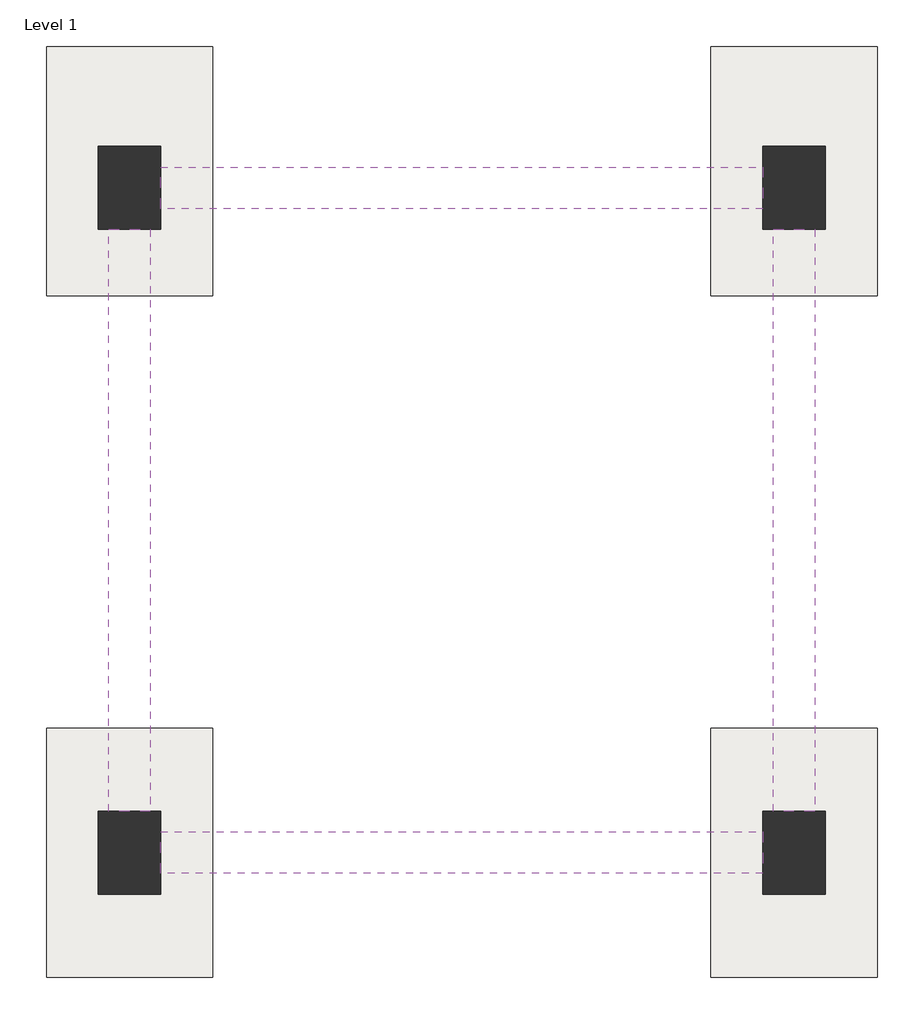
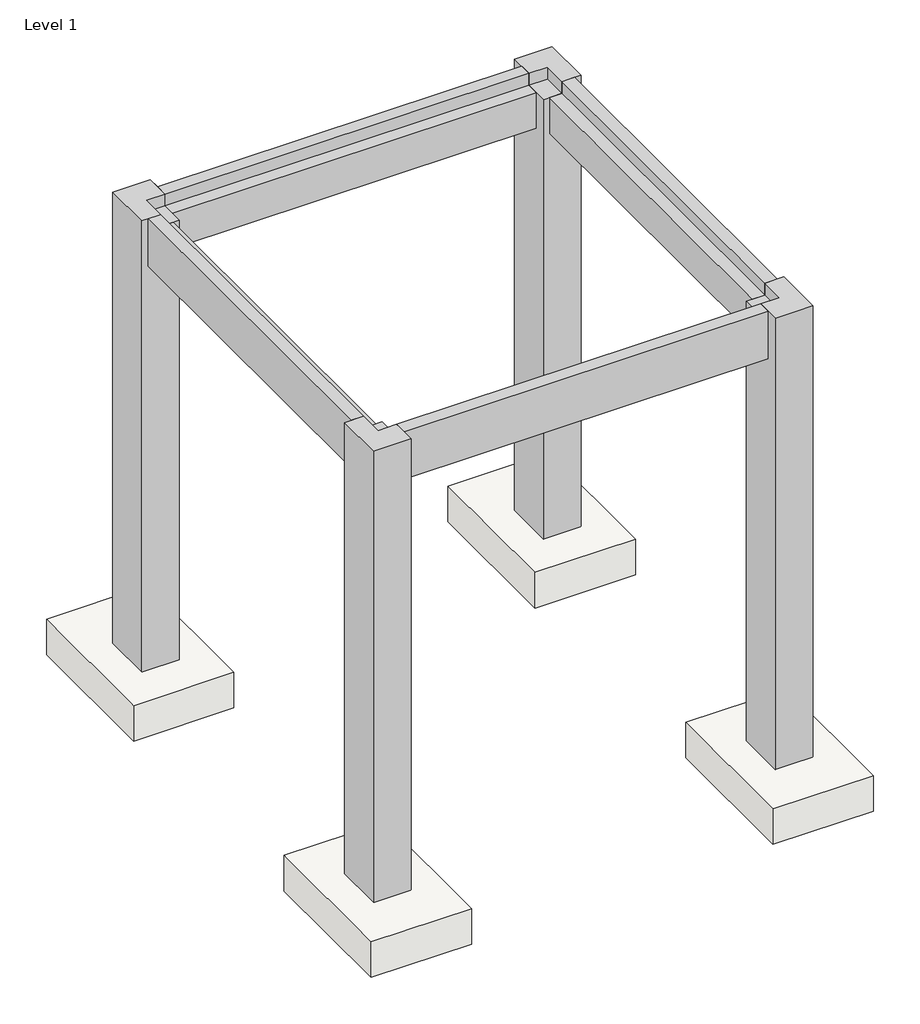
# One storey: 7 columns, 4 beams, 4 slabs.
"""IFC4 building model written with IfcOpenShell, lengths in millimetres."""

import ifcopenshell
import ifcopenshell.guid

model = None  # the IFC model being written
_history = None  # IfcOwnerHistory: only IFC2X3 demands one
_inside = {}  # id of a spatial element -> (the spatial element, [elements in it])
_under = {}  # id of a project, library or spatial element -> (it, [spatial elements below it])
_declared = {}  # id of a project -> (the project, [libraries it declares])
_typed = {}  # id of a type object -> (the type object, [elements of that type])
_made_of = {}  # id of a material, layer set ... -> (it, [elements and type objects made of it])


def new_model(schema):
    """Start an empty IFC model of exactly this schema.

    Asked for "IFC4X3", IfcOpenShell would pick the latest addendum, in which some entities
    have other attributes; the version numbers below select the first issue.
    IFC2X3 requires an IfcOwnerHistory on every rooted entity: one is made here for all.
    """
    global model, _history
    if schema == "IFC4X3":
        model = ifcopenshell.file(schema_version=(4, 3, 0, 0))
    else:
        model = ifcopenshell.file(schema=schema)
    _inside.clear()
    _under.clear()
    _declared.clear()
    _typed.clear()
    _made_of.clear()
    _history = None
    if model.schema == "IFC2X3":
        org = make("IfcOrganization", Name="unknown")
        user = make(
            "IfcPersonAndOrganization",
            ThePerson=make("IfcPerson", FamilyName="unknown"),
            TheOrganization=org,
        )
        app = make(
            "IfcApplication",
            ApplicationDeveloper=org,
            Version="unknown",
            ApplicationFullName="unknown",
            ApplicationIdentifier="unknown",
        )
        _history = make(
            "IfcOwnerHistory",
            OwningUser=user,
            OwningApplication=app,
            ChangeAction="ADDED",
            CreationDate=0,
        )
    return model


def make(cls, **values):
    """One entity of the class cls with the attributes given. An attribute that is None is left unset."""
    return model.create_entity(
        cls, **{name: value for name, value in values.items() if value is not None}
    )


def rooted(cls, **values):
    """An entity with a GlobalId (a new one), such as an element, a storey or a relation."""
    return make(cls, GlobalId=ifcopenshell.guid.new(), OwnerHistory=_history, **values)


def si_unit(unit_type, name, prefix=None):
    """IfcSIUnit, for example si_unit("LENGTHUNIT", "METRE", prefix="MILLI")."""
    return make("IfcSIUnit", UnitType=unit_type, Prefix=prefix, Name=name)


def assignment(units):
    """IfcUnitAssignment: the units of a project."""
    return None if units is None else make("IfcUnitAssignment", Units=units)


def point(xyz):
    """IfcCartesianPoint."""
    return None if xyz is None else make("IfcCartesianPoint", Coordinates=xyz)


def direction(xyz):
    """IfcDirection."""
    return None if xyz is None else make("IfcDirection", DirectionRatios=xyz)


def frame(location, z_axis=None, x_axis=None):
    """IfcAxis2Placement3D, a coordinate frame: its origin and axes. An axis left out is left unset."""
    return make(
        "IfcAxis2Placement3D",
        Location=point(location),
        Axis=direction(z_axis),
        RefDirection=direction(x_axis),
    )


def origin():
    """The frame at (0, 0, 0) with its axes left unset."""
    return frame((0.0, 0.0, 0.0))


def place(relative_to, where):
    """IfcLocalPlacement: puts the frame where relative to a parent placement (None: the world)."""
    return make(
        "IfcLocalPlacement", PlacementRelTo=relative_to, RelativePlacement=where
    )


def context(
    kind, dimensions, precision=None, world=None, true_north=None, identifier=None
):
    """IfcGeometricRepresentationContext, for example the 3D "Model" context."""
    return make(
        "IfcGeometricRepresentationContext",
        ContextIdentifier=identifier,
        ContextType=kind,
        CoordinateSpaceDimension=dimensions,
        Precision=precision,
        WorldCoordinateSystem=world,
        TrueNorth=true_north,
    )


def project(units=None, contexts=None):
    """IfcProject with its units and contexts."""
    return rooted(
        "IfcProject",
        Name="project",
        RepresentationContexts=contexts,
        UnitsInContext=assignment(units),
    )


def spatial(cls, under=None, at=None, **own):
    """A site, building, storey or space (cls), placed at a placement, below another one or the project."""
    s = rooted(cls, ObjectPlacement=at, **own)
    if under is not None:
        _under.setdefault(under.id(), (under, []))[1].append(s)
    return s


def polyline(points):
    """IfcPolyline through the points."""
    return make("IfcPolyline", Points=[point(p) for p in points])


def outline(outer, holes=None, kind="AREA"):
    """IfcArbitraryClosedProfileDef: a profile drawn as a closed curve; with holes, ...WithVoids."""
    if holes is None:
        return make("IfcArbitraryClosedProfileDef", ProfileType=kind, OuterCurve=outer)
    return make(
        "IfcArbitraryProfileDefWithVoids",
        ProfileType=kind,
        OuterCurve=outer,
        InnerCurves=holes,
    )


def extrude(swept, where, along, depth):
    """IfcExtrudedAreaSolid: the profile swept, set in the frame where, extruded along a direction by depth."""
    return make(
        "IfcExtrudedAreaSolid",
        SweptArea=swept,
        Position=where,
        ExtrudedDirection=direction(along),
        Depth=depth,
    )


def faces_of(points, faces, orient=None, outer=None):
    """IfcFace entities. A face is a list of loops; a loop is a list of indices into points, from 0.

    orient and outer hold one flag for each loop. By default every Orientation is true, the
    first loop of a face is its IfcFaceOuterBound and the others are IfcFaceBound.
    """
    made = []
    for i, loops in enumerate(faces):
        bounds = []
        for j, loop in enumerate(loops):
            is_outer = j == 0 if outer is None else outer[i][j]
            bounds.append(
                make(
                    "IfcFaceOuterBound" if is_outer else "IfcFaceBound",
                    Bound=make("IfcPolyLoop", Polygon=[points[k] for k in loop]),
                    Orientation=True if orient is None else orient[i][j],
                )
            )
        made.append(make("IfcFace", Bounds=bounds))
    return made


def faceted_brep(points, faces, orient=None, outer=None, voids=None):
    """IfcFacetedBrep: a solid bounded by flat faces; with voids (closed shells), ...WithVoids."""
    shared = [point(p) for p in points]
    hull = make("IfcClosedShell", CfsFaces=faces_of(shared, faces, orient, outer))
    if voids is None:
        return make("IfcFacetedBrep", Outer=hull)
    return make(
        "IfcFacetedBrepWithVoids",
        Outer=hull,
        Voids=[
            make(cls, CfsFaces=faces_of(shared, fs, o, b)) for cls, fs, o, b in voids
        ],
    )


def shape(context_of_items, identifier, shape_type, items):
    """IfcShapeRepresentation: the items that make up one representation, for example the "Body"."""
    return make(
        "IfcShapeRepresentation",
        ContextOfItems=context_of_items,
        RepresentationIdentifier=identifier,
        RepresentationType=shape_type,
        Items=items,
    )


def source(mapping_origin, context_of_items, identifier, shape_type, items):
    """IfcRepresentationMap: a shape defined once, which mapped items show again and again."""
    return make(
        "IfcRepresentationMap",
        MappingOrigin=mapping_origin,
        MappedRepresentation=shape(context_of_items, identifier, shape_type, items),
    )


def transform(
    local_origin,
    x_axis=None,
    y_axis=None,
    z_axis=None,
    scale=None,
    scale2=None,
    scale3=None,
    uniform=True,
):
    """IfcCartesianTransformationOperator3D, or its non-uniform kind. x_axis, y_axis, z_axis: its Axis1, 2, 3."""
    if uniform:
        return make(
            "IfcCartesianTransformationOperator3D",
            Axis1=direction(x_axis),
            Axis2=direction(y_axis),
            LocalOrigin=point(local_origin),
            Scale=scale,
            Axis3=direction(z_axis),
        )
    return make(
        "IfcCartesianTransformationOperator3DnonUniform",
        Axis1=direction(x_axis),
        Axis2=direction(y_axis),
        LocalOrigin=point(local_origin),
        Scale=scale,
        Axis3=direction(z_axis),
        Scale2=scale2,
        Scale3=scale3,
    )


def mapped(mapping_source, mapping_target):
    """IfcMappedItem: shows the shape of a source again, moved by a transform."""
    return make(
        "IfcMappedItem", MappingSource=mapping_source, MappingTarget=mapping_target
    )


def made_of(thing, what):
    """Note that an element or type object is made of a material, layer set ...; save() writes the relation."""
    if what is not None:
        _made_of.setdefault(what.id(), (what, []))[1].append(thing)
    return thing


def element(
    cls,
    number,
    at=None,
    inside=None,
    cuts=None,
    type_object=None,
    material=None,
    context=None,
    identifier="Body",
    shape_type=None,
    held_by="IfcProductDefinitionShape",
    body=None,
    shapes=None,
    **own,
):
    """One element of the class cls, such as IfcWall. Its Tag is "e" and its number.

    at: its placement. inside: the storey or other place that contains it. cuts: it is an
    opening in that element (IfcRelVoidsElement). A single representation is given by context,
    identifier, shape_type and body (its items); several are given by shapes. held_by: the class
    of the entity that holds the representations. save() writes the other relations.
    """
    e = rooted(cls, Tag="e%d" % number, ObjectPlacement=at, **own)
    if body is not None:
        shapes = [shape(context, identifier, shape_type, body)]
    if shapes is not None:
        e.Representation = make(held_by, Representations=shapes)
    if inside is not None:
        _inside.setdefault(inside.id(), (inside, []))[1].append(e)
    if cuts is not None:
        rooted(
            "IfcRelVoidsElement", RelatingBuildingElement=cuts, RelatedOpeningElement=e
        )
    if type_object is not None:
        _typed.setdefault(type_object.id(), (type_object, []))[1].append(e)
    return made_of(e, material)


def aggregate(whole, parts):
    """IfcRelAggregates: a whole, such as a stair, and the parts it consists of."""
    return rooted("IfcRelAggregates", RelatingObject=whole, RelatedObjects=parts)


def save(model, path):
    """Write the relations noted so far, then the file.

    IfcRelAggregates (storeys below a building ...), IfcRelContainedInSpatialStructure (elements
    in a storey), IfcRelDefinesByType, IfcRelAssociatesMaterial and IfcRelDeclares: one each for
    every whole, place, type object, material and project.
    """
    for whole, parts in _under.values():
        aggregate(whole, parts)
    for where, things in _inside.values():
        rooted(
            "IfcRelContainedInSpatialStructure",
            RelatedElements=things,
            RelatingStructure=where,
        )
    for kind, things in _typed.values():
        rooted("IfcRelDefinesByType", RelatedObjects=things, RelatingType=kind)
    for what, things in _made_of.values():
        rooted("IfcRelAssociatesMaterial", RelatedObjects=things, RelatingMaterial=what)
    for by, libraries in _declared.values():
        rooted("IfcRelDeclares", RelatingContext=by, RelatedDefinitions=libraries)
    model.write(path)


def slab_5ba74754(model_context):
    return source(origin(), model_context, "Body", "SweptSolid", [
        extrude(outline(polyline([(609.6, 914.4), (609.6, -914.4), (-609.6, -914.4), (-609.6, 914.4), (609.6, 914.4)])), frame((0.0, 0.0, -457.2), z_axis=(0.0, 0.0, 1.0), x_axis=(1.0, 0.0, 0.0)), (0.0, 0.0, 1.0), 457.2),
    ])


model = new_model("IFC4")

# Units and contexts
model_context = context("Model", 3, world=origin())
ifc_project = project(units=[si_unit("LENGTHUNIT", "METRE", prefix="MILLI")], contexts=[model_context])

# Site, building, storey
site = spatial("IfcSite", under=ifc_project)
building = spatial("IfcBuilding", under=site)
storey = spatial("IfcBuildingStorey", under=building, Name="Level 1", Elevation=0.0)

# Beams
placement = place(None, origin())
element("IfcBeam", 1, ObjectType="Concrete-Rectangular Beam : 12 x 24", at=placement, inside=storey, context=model_context, shape_type="SweptSolid", body=[
    extrude(outline(polyline([(786.0323826, 2438.4), (786.0323826, 3048.0), (938.4323826, 3048.0), (938.4323826, 2895.6), (1090.8323826, 2895.6), (1090.8323826, 2438.4), (786.0323826, 2438.4)])), frame((-11045.0800525, 0.0, 0.0), z_axis=(1.0, 0.0, 0.0), x_axis=(0.0, 1.0, 0.0)), (0.0, 0.0, 1.0), 4419.6),
])
element("IfcBeam", 2, ObjectType="Concrete-Rectangular Beam : 12 x 24", at=placement, inside=storey, context=model_context, shape_type="SweptSolid", body=[
    extrude(outline(polyline([(5967.6323826, 3048.0), (5967.6323826, 2438.4), (5662.8323826, 2438.4), (5662.8323826, 2895.6), (5815.2323826, 2895.6), (5815.2323826, 3048.0), (5967.6323826, 3048.0)])), frame((-11045.0800525, 0.0, 0.0), z_axis=(1.0, 0.0, 0.0), x_axis=(0.0, 1.0, 0.0)), (0.0, 0.0, 1.0), 4419.6),
])
element("IfcBeam", 3, ObjectType="Concrete-Rectangular Beam : 12 x 24", at=placement, inside=storey, context=model_context, shape_type="SweptSolid", body=[
    extrude(outline(polyline([(2438.4, -11426.0800525), (2438.4, -11121.2800525), (2895.6, -11121.2800525), (2895.6, -11273.6800525), (3048.0, -11273.6800525), (3048.0, -11426.0800525), (2438.4, -11426.0800525)])), frame((0.0, 1243.2323826, 0.0), z_axis=(0.0, 1.0, 0.0), x_axis=(0.0, 0.0, 1.0)), (0.0, 0.0, 1.0), 4267.2),
])
element("IfcBeam", 4, ObjectType="Concrete-Rectangular Beam : 12 x 24", at=placement, inside=storey, context=model_context, shape_type="SweptSolid", body=[
    extrude(outline(polyline([(2438.4, -6244.4800525), (3048.0, -6244.4800525), (3048.0, -6396.8800525), (2895.6, -6396.8800525), (2895.6, -6549.2800525), (2438.4, -6549.2800525), (2438.4, -6244.4800525)])), frame((0.0, 1243.2323826, 0.0), z_axis=(0.0, 1.0, 0.0), x_axis=(0.0, 0.0, 1.0)), (0.0, 0.0, 1.0), 4267.2),
])

# Columns
element("IfcColumn", 5, ObjectType="Concrete-Rectangular-Column : 18 x 24", at=placement, inside=storey, context=model_context, shape_type="Brep", body=[
    faceted_brep([(-11045.0800525, 6120.0323826, 3048.0), (-11502.2800525, 6120.0323826, 3048.0), (-11502.2800525, 5510.4323826, 3048.0), (-11273.6800525, 5510.4323826, 3048.0), (-11273.6800525, 5815.2323826, 3048.0), (-11045.0800525, 5815.2323826, 3048.0), (-11045.0800525, 6120.0323826, -2743.2), (-11045.0800525, 5510.4323826, -2743.2), (-11502.2800525, 5510.4323826, -2743.2), (-11502.2800525, 6120.0323826, -2743.2), (-11045.0800525, 5510.4323826, 2895.6), (-11273.6800525, 5510.4323826, 2895.6), (-11045.0800525, 5815.2323826, 2895.6), (-11273.6800525, 5815.2323826, 2895.6)], [[[0, 1, 2, 3, 4, 5]], [[6, 7, 8, 9]], [[1, 0, 6, 9]], [[2, 1, 9, 8]], [[8, 7, 10, 11, 3, 2]], [[7, 6, 0, 5, 12, 10]], [[13, 11, 10, 12]], [[4, 13, 12, 5]], [[13, 4, 3, 11]]]),
])
element("IfcColumn", 6, ObjectType="Concrete-Rectangular-Column : 18 x 24", at=placement, inside=storey, context=model_context, shape_type="Brep", body=[
    faceted_brep([(-6168.2800525, 6120.0323826, 3048.0), (-6625.4800525, 6120.0323826, 3048.0), (-6625.4800525, 5815.2323826, 3048.0), (-6396.8800525, 5815.2323826, 3048.0), (-6396.8800525, 5510.4323826, 3048.0), (-6168.2800525, 5510.4323826, 3048.0), (-6168.2800525, 6120.0323826, -2743.2), (-6168.2800525, 5510.4323826, -2743.2), (-6625.4800525, 5510.4323826, -2743.2), (-6625.4800525, 6120.0323826, -2743.2), (-6625.4800525, 5510.4323826, 2895.6), (-6625.4800525, 5815.2323826, 2895.6), (-6396.8800525, 5510.4323826, 2895.6), (-6396.8800525, 5815.2323826, 2895.6)], [[[0, 1, 2, 3, 4, 5]], [[6, 7, 8, 9]], [[1, 0, 6, 9]], [[9, 8, 10, 11, 2, 1]], [[8, 7, 5, 4, 12, 10]], [[0, 5, 7, 6]], [[12, 13, 11, 10]], [[13, 3, 2, 11]], [[3, 13, 12, 4]]]),
])
element("IfcColumn", 7, ObjectType="Concrete-Rectangular-Column : 18 x 24", at=placement, inside=storey, context=model_context, shape_type="Brep", body=[
    faceted_brep([(-11045.0800525, 6120.0323826, 3048.0), (-11502.2800525, 6120.0323826, 3048.0), (-11502.2800525, 5510.4323826, 3048.0), (-11426.0800525, 5510.4323826, 3048.0), (-11273.6800525, 5510.4323826, 3048.0), (-11273.6800525, 5815.2323826, 3048.0), (-11045.0800525, 5815.2323826, 3048.0), (-11045.0800525, 5967.6323826, 3048.0), (-11045.0800525, 6120.0323826, -2743.2), (-11045.0800525, 5510.4323826, -2743.2), (-11502.2800525, 5510.4323826, -2743.2), (-11502.2800525, 6120.0323826, -2743.2), (-11045.0800525, 5510.4323826, 2895.6), (-11121.2800525, 5510.4323826, 2895.6), (-11273.6800525, 5510.4323826, 2895.6), (-11045.0800525, 5815.2323826, 2895.6), (-11045.0800525, 5662.8323826, 2895.6), (-11273.6800525, 5815.2323826, 2895.6)], [[[0, 1, 2, 3, 4, 5, 6, 7]], [[8, 9, 10, 11]], [[1, 0, 8, 11]], [[2, 1, 11, 10]], [[10, 9, 12, 13, 14, 4, 3, 2]], [[9, 8, 0, 7, 6, 15, 16, 12]], [[17, 14, 13, 12, 16, 15]], [[5, 17, 15, 6]], [[17, 5, 4, 14]]]),
])
element("IfcColumn", 8, ObjectType="Concrete-Rectangular-Column : 18 x 24", at=placement, inside=storey, context=model_context, shape_type="Brep", body=[
    faceted_brep([(-11045.0800525, 6120.0323826, 3048.0), (-11502.2800525, 6120.0323826, 3048.0), (-11502.2800525, 5510.4323826, 3048.0), (-11426.0800525, 5510.4323826, 3048.0), (-11273.6800525, 5510.4323826, 3048.0), (-11273.6800525, 5815.2323826, 3048.0), (-11045.0800525, 5815.2323826, 3048.0), (-11045.0800525, 5967.6323826, 3048.0), (-11045.0800525, 6120.0323826, -2743.2), (-11045.0800525, 5510.4323826, -2743.2), (-11502.2800525, 5510.4323826, -2743.2), (-11502.2800525, 6120.0323826, -2743.2), (-11045.0800525, 5510.4323826, 2895.6), (-11121.2800525, 5510.4323826, 2895.6), (-11273.6800525, 5510.4323826, 2895.6), (-11045.0800525, 5815.2323826, 2895.6), (-11045.0800525, 5662.8323826, 2895.6), (-11273.6800525, 5815.2323826, 2895.6)], [[[0, 1, 2, 3, 4, 5, 6, 7]], [[8, 9, 10, 11]], [[1, 0, 8, 11]], [[2, 1, 11, 10]], [[10, 9, 12, 13, 14, 4, 3, 2]], [[9, 8, 0, 7, 6, 15, 16, 12]], [[17, 14, 13, 12, 16, 15]], [[5, 17, 15, 6]], [[17, 5, 4, 14]]]),
])
element("IfcColumn", 9, ObjectType="Concrete-Rectangular-Column : 18 x 24", at=placement, inside=storey, context=model_context, shape_type="Brep", body=[
    faceted_brep([(-11045.0800525, 6120.0323826, 3048.0), (-11502.2800525, 6120.0323826, 3048.0), (-11502.2800525, 5510.4323826, 3048.0), (-11426.0800525, 5510.4323826, 3048.0), (-11273.6800525, 5510.4323826, 3048.0), (-11273.6800525, 5815.2323826, 3048.0), (-11045.0800525, 5815.2323826, 3048.0), (-11045.0800525, 5967.6323826, 3048.0), (-11045.0800525, 6120.0323826, -2743.2), (-11045.0800525, 5510.4323826, -2743.2), (-11502.2800525, 5510.4323826, -2743.2), (-11502.2800525, 6120.0323826, -2743.2), (-11045.0800525, 5510.4323826, 2895.6), (-11121.2800525, 5510.4323826, 2895.6), (-11273.6800525, 5510.4323826, 2895.6), (-11045.0800525, 5815.2323826, 2895.6), (-11045.0800525, 5662.8323826, 2895.6), (-11273.6800525, 5815.2323826, 2895.6)], [[[0, 1, 2, 3, 4, 5, 6, 7]], [[8, 9, 10, 11]], [[1, 0, 8, 11]], [[2, 1, 11, 10]], [[10, 9, 12, 13, 14, 4, 3, 2]], [[9, 8, 0, 7, 6, 15, 16, 12]], [[17, 14, 13, 12, 16, 15]], [[5, 17, 15, 6]], [[17, 5, 4, 14]]]),
])
element("IfcColumn", 10, ObjectType="Concrete-Rectangular-Column : 18 x 24", at=placement, inside=storey, context=model_context, shape_type="Brep", body=[
    faceted_brep([(-11502.2800525, 1243.2323826, 3048.0), (-11502.2800525, 633.6323826, 3048.0), (-11045.0800525, 633.6323826, 3048.0), (-11045.0800525, 938.4323826, 3048.0), (-11273.6800525, 938.4323826, 3048.0), (-11273.6800525, 1243.2323826, 3048.0), (-11045.0800525, 1243.2323826, -2743.2), (-11045.0800525, 633.6323826, -2743.2), (-11502.2800525, 633.6323826, -2743.2), (-11502.2800525, 1243.2323826, -2743.2), (-11273.6800525, 1243.2323826, 2895.6), (-11045.0800525, 1243.2323826, 2895.6), (-11045.0800525, 938.4323826, 2895.6), (-11273.6800525, 938.4323826, 2895.6)], [[[0, 1, 2, 3, 4, 5]], [[6, 7, 8, 9]], [[6, 9, 0, 5, 10, 11]], [[1, 0, 9, 8]], [[2, 1, 8, 7]], [[7, 6, 11, 12, 3, 2]], [[10, 13, 12, 11]], [[13, 4, 3, 12]], [[4, 13, 10, 5]]]),
])
element("IfcColumn", 11, ObjectType="Concrete-Rectangular-Column : 18 x 24", at=placement, inside=storey, context=model_context, shape_type="Brep", body=[
    faceted_brep([(-6625.4800525, 633.6323826, 3048.0), (-6168.2800525, 633.6323826, 3048.0), (-6168.2800525, 1243.2323826, 3048.0), (-6396.8800525, 1243.2323826, 3048.0), (-6396.8800525, 938.4323826, 3048.0), (-6625.4800525, 938.4323826, 3048.0), (-6168.2800525, 1243.2323826, -2743.2), (-6168.2800525, 633.6323826, -2743.2), (-6625.4800525, 633.6323826, -2743.2), (-6625.4800525, 1243.2323826, -2743.2), (-6625.4800525, 1243.2323826, 2895.6), (-6396.8800525, 1243.2323826, 2895.6), (-6625.4800525, 938.4323826, 2895.6), (-6396.8800525, 938.4323826, 2895.6)], [[[0, 1, 2, 3, 4, 5]], [[6, 7, 8, 9]], [[6, 9, 10, 11, 3, 2]], [[9, 8, 0, 5, 12, 10]], [[1, 0, 8, 7]], [[2, 1, 7, 6]], [[12, 13, 11, 10]], [[13, 4, 3, 11]], [[4, 13, 12, 5]]]),
])

# Slabs
slab_shape = slab_5ba74754(model_context)
element("IfcSlab", 12, ObjectType="Footing-Rectangular : 72\" x 48\" x 18\"", at=placement, inside=storey, context=model_context, shape_type="MappedRepresentation", body=[
    mapped(slab_shape, transform((-11273.6800525, 5938.4323826, -2743.2), x_axis=(1.0, 0.0, 0.0), y_axis=(0.0, 1.0, 0.0), z_axis=(0.0, 0.0, 1.0))),
])
element("IfcSlab", 13, ObjectType="Footing-Rectangular : 72\" x 48\" x 18\"", at=placement, inside=storey, context=model_context, shape_type="MappedRepresentation", body=[
    mapped(slab_shape, transform((-6396.8800525, 5938.4323826, -2743.2), x_axis=(1.0, 0.0, 0.0), y_axis=(0.0, 1.0, 0.0), z_axis=(0.0, 0.0, 1.0))),
])
element("IfcSlab", 14, ObjectType="Footing-Rectangular : 72\" x 48\" x 18\"", at=placement, inside=storey, context=model_context, shape_type="MappedRepresentation", body=[
    mapped(slab_shape, transform((-11273.6800525, 938.4323826, -2743.2), x_axis=(1.0, 0.0, 0.0), y_axis=(0.0, 1.0, 0.0), z_axis=(0.0, 0.0, 1.0))),
])
element("IfcSlab", 15, ObjectType="Footing-Rectangular : 72\" x 48\" x 18\"", at=placement, inside=storey, context=model_context, shape_type="MappedRepresentation", body=[
    mapped(slab_shape, transform((-6396.8800525, 938.4323826, -2743.2), x_axis=(1.0, 0.0, 0.0), y_axis=(0.0, 1.0, 0.0), z_axis=(0.0, 0.0, 1.0))),
])

save(model, "model.ifc")

# Revit data of these elements
# Project information
#   Project Issue Date = "Issue Date"
#   Project Status = "Project Status"
#   Client Name = "Owner"
#   Project Address = "Enter address here"
#   Project Name = "Project Name"
#   Project Number = "Project Number"
# Grids (mm)
#   "1": line (9019.216, 5815.232) -> (-21563.036, 5815.232)
#   "2": line (-11273.68, -9686.145) -> (-11273.68, 17085.235)
#   "3": line (-6396.88, 17085.235) -> (-6396.88, -9686.145)
#   "4.78": line (9019.216, 938.432) -> (-21563.036, 938.432)
# Type "Concrete-Rectangular Beam : 12 x 24"
#   Assembly Code = "B10"
#   Length [instance default] = 1.524 m
#   b = 0.3048 m
#   h = 0.6096 m
#   Structural Material [instance default] = Concrete - Cast-in-Place Concrete
# Type "Concrete-Rectangular-Column : 18 x 24"
#   Assembly Code = "B10"
#   b = 0.4572 m
#   h = 0.6096 m
#   Structural Material [instance default] = Concrete - Cast-in-Place Concrete
# Type "Footing-Rectangular : 72\" x 48\" x 18\""
#   Assembly Code = "A1010100"
#   Width = 1.2192 m
#   Length = 1.8288 m
#   Thickness = 0.4572 m
#   Structural Material [instance default] = Concrete - Cast-in-Place Concrete
# Elements 1, 2, 3, 4 (IfcBeam, "Concrete-Rectangular Beam : 12 x 24")
#   Comments = ""
#   Structural Material = Concrete - Cast-in-Place Concrete
#   Phase Created = New Construction
#   Materials on its faces: "Concrete - Cast-in-Place Concrete"
# Elements 5, 6, 7, 8, 9, 10, 11 (IfcColumn, "Concrete-Rectangular-Column : 18 x 24")
#   Structural Material = Concrete - Cast-in-Place Concrete
#   Phase Created = New Construction
#   Materials on its faces: "Concrete - Cast-in-Place Concrete"
# Element 12 (IfcSlab, "Footing-Rectangular : 72\" x 48\" x 18\"")
#   Structural Material = Concrete - Cast-in-Place Concrete
#   Phase Created = New Construction
#   Materials on its faces: "Concrete - Cast-in-Place Concrete"
# Elements 13, 14, 15 (IfcSlab, "Footing-Rectangular : 72\" x 48\" x 18\"")
#   Comments = ""
#   Structural Material = Concrete - Cast-in-Place Concrete
#   Phase Created = New Construction
#   Materials on its faces: "Concrete - Cast-in-Place Concrete"
# Materials
#   "Concrete - Cast-in-Place Concrete": class "Concrete", colour RGB 192 192 192, transparency 0
